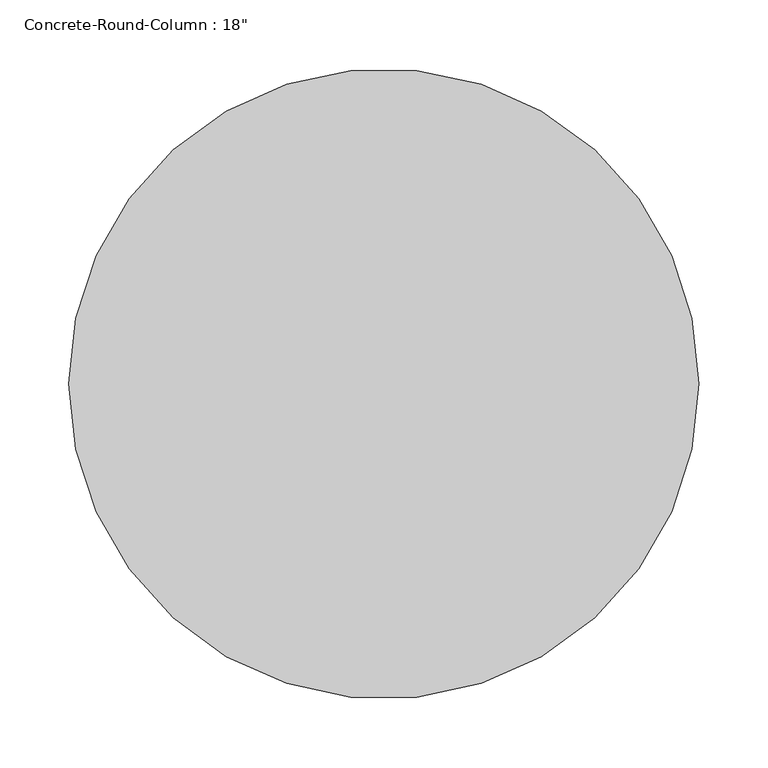
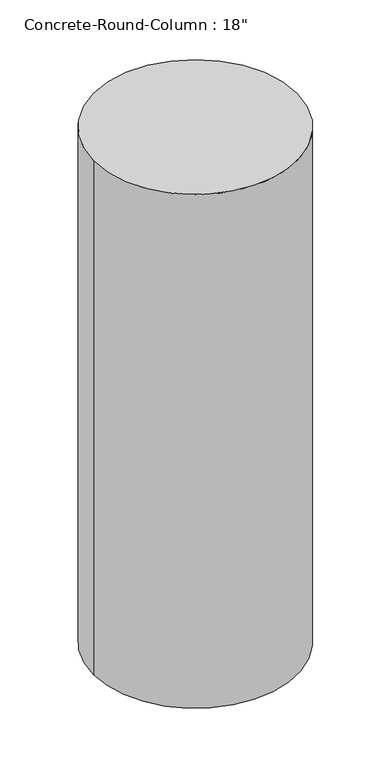
"""IFC4 building model written with IfcOpenShell, lengths in millimetres: column geometry."""

from ifc_helpers import new_model, si_unit, point, frame, origin, origin_2d, place, context, project, spatial, circle_curve, trimmed, segment, composite_curve, outline, extrude, source, transform, mapped, element, save


def column_c9326fad(model_context):
    return source(origin(), model_context, "Body", "SweptSolid", [
        extrude(outline(composite_curve([segment(trimmed(circle_curve(origin_2d(), 228.6), [point((-228.6, 0.0))], [point((228.6, 0.0))], False, "CARTESIAN"), True, "CONTINUOUS"), segment(trimmed(circle_curve(origin_2d(), 228.6), [point((228.6, 0.0))], [point((-228.6, 0.0))], False, "CARTESIAN"), True, "CONTINUOUS")], self_intersect=False)), frame((0.0, 0.0, 262820.15), z_axis=(0.0, 0.0, 1.0), x_axis=(1.0, 0.0, 0.0)), (0.0, 0.0, 1.0), 1219.2),
    ])


if __name__ == "__main__":
    model = new_model("IFC4")
    model_context = context("Model", 3, world=origin())
    ifc_project = project(units=[si_unit("LENGTHUNIT", "METRE", prefix="MILLI")], contexts=[model_context])
    site = spatial("IfcSite", under=ifc_project)
    building = spatial("IfcBuilding", under=site)
    placement = place(None, origin())
    column_shape = column_c9326fad(model_context)
    element("IfcColumn", 1, ObjectType="Concrete-Round-Column : 18\"", at=placement, inside=building, context=model_context, shape_type="MappedRepresentation", body=[
        mapped(column_shape, transform((0.0, 0.0, 0.0), x_axis=(1.0, 0.0, 0.0), y_axis=(0.0, 1.0, 0.0), z_axis=(0.0, 0.0, 1.0))),
    ])
    save(model, "model.ifc")

# Revit data of these elements
# Type "Concrete-Round-Column : 18\""
#   Assembly Code = "B10"
#   b = 1' - 6"
#   Structural Material [instance default] = Concrete, Cast-in-Place gray
# Element 1 (IfcColumn, "Concrete-Round-Column : 18\"")
#   Materials on its faces: "Concrete, Cast-in-Place gray"
# Materials
#   "Concrete, Cast-in-Place gray": class "Concrete", colour RGB 110 111 103, transparency 0, Description = "Cast-in-place concrete", Cost = 0
